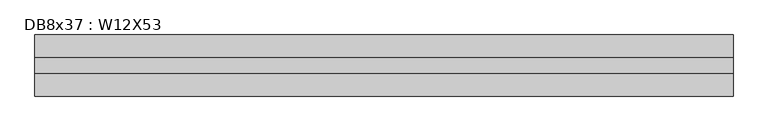
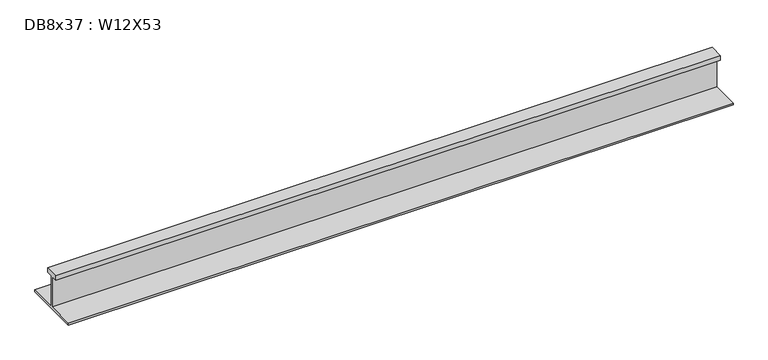
"""IFC4 building model written with IfcOpenShell, lengths in millimetres: beam geometry, DB8x37 : W12X53."""

from ifc_helpers import new_model, si_unit, frame, origin, place, context, project, spatial, polyline, outline, extrude, source, transform, mapped, element, save


def db8x37_w12x53_8667b28d(model_context):
    return source(origin(), model_context, "Body", "SweptSolid", [
        extrude(outline(polyline([(38.1, 145.415), (38.1, 120.015), (2.921, 120.015), (2.921, -48.4505), (152.4, -48.4505), (152.4, -58.1025), (-152.4, -58.1025), (-152.4, -48.4505), (-2.921, -48.4505), (-2.921, 120.015), (-38.1, 120.015), (-38.1, 145.415), (38.1, 145.415)])), frame((-1679.829, 0.0, 0.0), z_axis=(1.0, 0.0, 0.0), x_axis=(0.0, 1.0, 0.0)), (0.0, 0.0, 1.0), 3483.2289994),
    ])


if __name__ == "__main__":
    model = new_model("IFC4")
    model_context = context("Model", 3, world=origin())
    ifc_project = project(units=[si_unit("LENGTHUNIT", "METRE", prefix="MILLI")], contexts=[model_context])
    site = spatial("IfcSite", under=ifc_project)
    building = spatial("IfcBuilding", under=site)
    placement = place(None, origin())
    db8x37_w12x53_shape = db8x37_w12x53_8667b28d(model_context)
    element("IfcBeam", 1, ObjectType="DB8x37 : W12X53", at=placement, inside=building, context=model_context, shape_type="MappedRepresentation", body=[
        mapped(db8x37_w12x53_shape, transform((0.0, 0.0, 0.0), x_axis=(1.0, 0.0, 0.0), y_axis=(0.0, 1.0, 0.0), z_axis=(0.0, 0.0, 1.0))),
    ])
    save(model, "model.ifc")

# Revit data of these elements
# Type "DB8x37 : W12X53"
#   Assembly Code = "B10"
#   W = 53
#   Length [instance default] = 5' - 0"
#   bf = 0' - 10"
#   d = 1' - 0.1"
#   k = 0' - 1 3/8"
#   k2 = 0' - 0.8"
#   tf = 0' - 0.575"
#   tw = 0' - 0.345"
#   A = 0.108333 SF
#   Structural Material [instance default] = Steel ASTM A992
# Element 1 (IfcBeam, "DB8x37 : W12X53")
#   Materials on its faces: "Steel ASTM A992"
# Materials
#   "Steel ASTM A992": class "Metal", colour RGB 199 199 199, transparency 0, Description = "Structural steel 50ksi", Cost = 0
